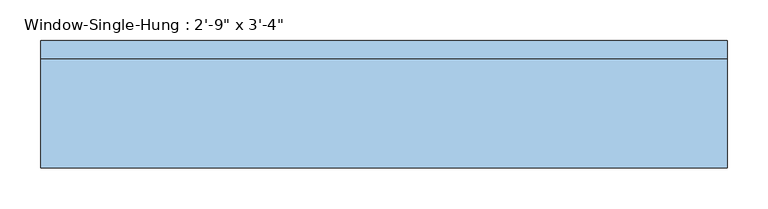
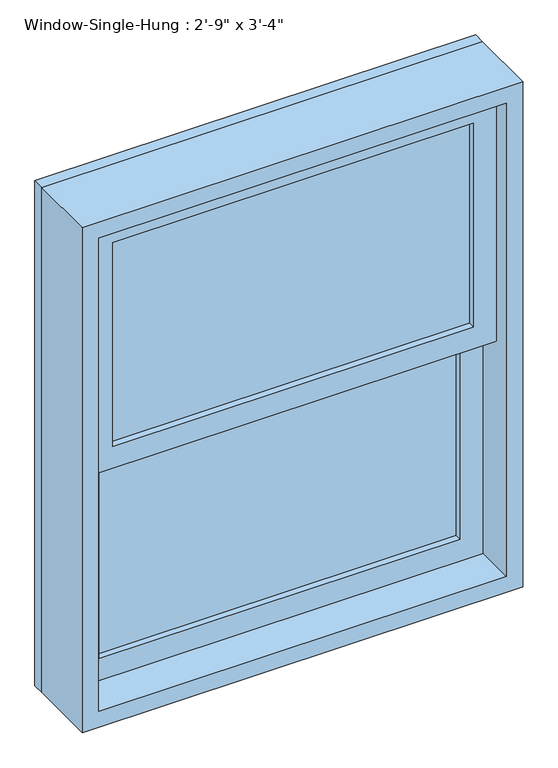
"""IFC4 building model written with IfcOpenShell, lengths in millimetres: window geometry."""

import ifcopenshell
import ifcopenshell.guid

model = None  # the IFC model being written
_history = None  # IfcOwnerHistory: only IFC2X3 demands one
_inside = {}  # id of a spatial element -> (the spatial element, [elements in it])
_under = {}  # id of a project, library or spatial element -> (it, [spatial elements below it])
_declared = {}  # id of a project -> (the project, [libraries it declares])
_typed = {}  # id of a type object -> (the type object, [elements of that type])
_made_of = {}  # id of a material, layer set ... -> (it, [elements and type objects made of it])


def new_model(schema):
    """Start an empty IFC model of exactly this schema.

    Asked for "IFC4X3", IfcOpenShell would pick the latest addendum, in which some entities
    have other attributes; the version numbers below select the first issue.
    IFC2X3 requires an IfcOwnerHistory on every rooted entity: one is made here for all.
    """
    global model, _history
    if schema == "IFC4X3":
        model = ifcopenshell.file(schema_version=(4, 3, 0, 0))
    else:
        model = ifcopenshell.file(schema=schema)
    _inside.clear()
    _under.clear()
    _declared.clear()
    _typed.clear()
    _made_of.clear()
    _history = None
    if model.schema == "IFC2X3":
        org = make("IfcOrganization", Name="unknown")
        user = make(
            "IfcPersonAndOrganization",
            ThePerson=make("IfcPerson", FamilyName="unknown"),
            TheOrganization=org,
        )
        app = make(
            "IfcApplication",
            ApplicationDeveloper=org,
            Version="unknown",
            ApplicationFullName="unknown",
            ApplicationIdentifier="unknown",
        )
        _history = make(
            "IfcOwnerHistory",
            OwningUser=user,
            OwningApplication=app,
            ChangeAction="ADDED",
            CreationDate=0,
        )
    return model


def make(cls, **values):
    """One entity of the class cls with the attributes given. An attribute that is None is left unset."""
    return model.create_entity(
        cls, **{name: value for name, value in values.items() if value is not None}
    )


def rooted(cls, **values):
    """An entity with a GlobalId (a new one), such as an element, a storey or a relation."""
    return make(cls, GlobalId=ifcopenshell.guid.new(), OwnerHistory=_history, **values)


def si_unit(unit_type, name, prefix=None):
    """IfcSIUnit, for example si_unit("LENGTHUNIT", "METRE", prefix="MILLI")."""
    return make("IfcSIUnit", UnitType=unit_type, Prefix=prefix, Name=name)


def assignment(units):
    """IfcUnitAssignment: the units of a project."""
    return None if units is None else make("IfcUnitAssignment", Units=units)


def point(xyz):
    """IfcCartesianPoint."""
    return None if xyz is None else make("IfcCartesianPoint", Coordinates=xyz)


def direction(xyz):
    """IfcDirection."""
    return None if xyz is None else make("IfcDirection", DirectionRatios=xyz)


def frame(location, z_axis=None, x_axis=None):
    """IfcAxis2Placement3D, a coordinate frame: its origin and axes. An axis left out is left unset."""
    return make(
        "IfcAxis2Placement3D",
        Location=point(location),
        Axis=direction(z_axis),
        RefDirection=direction(x_axis),
    )


def origin():
    """The frame at (0, 0, 0) with its axes left unset."""
    return frame((0.0, 0.0, 0.0))


def place(relative_to, where):
    """IfcLocalPlacement: puts the frame where relative to a parent placement (None: the world)."""
    return make(
        "IfcLocalPlacement", PlacementRelTo=relative_to, RelativePlacement=where
    )


def context(
    kind, dimensions, precision=None, world=None, true_north=None, identifier=None
):
    """IfcGeometricRepresentationContext, for example the 3D "Model" context."""
    return make(
        "IfcGeometricRepresentationContext",
        ContextIdentifier=identifier,
        ContextType=kind,
        CoordinateSpaceDimension=dimensions,
        Precision=precision,
        WorldCoordinateSystem=world,
        TrueNorth=true_north,
    )


def project(units=None, contexts=None):
    """IfcProject with its units and contexts."""
    return rooted(
        "IfcProject",
        Name="project",
        RepresentationContexts=contexts,
        UnitsInContext=assignment(units),
    )


def spatial(cls, under=None, at=None, **own):
    """A site, building, storey or space (cls), placed at a placement, below another one or the project."""
    s = rooted(cls, ObjectPlacement=at, **own)
    if under is not None:
        _under.setdefault(under.id(), (under, []))[1].append(s)
    return s


def polyline(points):
    """IfcPolyline through the points."""
    return make("IfcPolyline", Points=[point(p) for p in points])


def outline(outer, holes=None, kind="AREA"):
    """IfcArbitraryClosedProfileDef: a profile drawn as a closed curve; with holes, ...WithVoids."""
    if holes is None:
        return make("IfcArbitraryClosedProfileDef", ProfileType=kind, OuterCurve=outer)
    return make(
        "IfcArbitraryProfileDefWithVoids",
        ProfileType=kind,
        OuterCurve=outer,
        InnerCurves=holes,
    )


def extrude(swept, where, along, depth):
    """IfcExtrudedAreaSolid: the profile swept, set in the frame where, extruded along a direction by depth."""
    return make(
        "IfcExtrudedAreaSolid",
        SweptArea=swept,
        Position=where,
        ExtrudedDirection=direction(along),
        Depth=depth,
    )


def shape(context_of_items, identifier, shape_type, items):
    """IfcShapeRepresentation: the items that make up one representation, for example the "Body"."""
    return make(
        "IfcShapeRepresentation",
        ContextOfItems=context_of_items,
        RepresentationIdentifier=identifier,
        RepresentationType=shape_type,
        Items=items,
    )


def source(mapping_origin, context_of_items, identifier, shape_type, items):
    """IfcRepresentationMap: a shape defined once, which mapped items show again and again."""
    return make(
        "IfcRepresentationMap",
        MappingOrigin=mapping_origin,
        MappedRepresentation=shape(context_of_items, identifier, shape_type, items),
    )


def transform(
    local_origin,
    x_axis=None,
    y_axis=None,
    z_axis=None,
    scale=None,
    scale2=None,
    scale3=None,
    uniform=True,
):
    """IfcCartesianTransformationOperator3D, or its non-uniform kind. x_axis, y_axis, z_axis: its Axis1, 2, 3."""
    if uniform:
        return make(
            "IfcCartesianTransformationOperator3D",
            Axis1=direction(x_axis),
            Axis2=direction(y_axis),
            LocalOrigin=point(local_origin),
            Scale=scale,
            Axis3=direction(z_axis),
        )
    return make(
        "IfcCartesianTransformationOperator3DnonUniform",
        Axis1=direction(x_axis),
        Axis2=direction(y_axis),
        LocalOrigin=point(local_origin),
        Scale=scale,
        Axis3=direction(z_axis),
        Scale2=scale2,
        Scale3=scale3,
    )


def mapped(mapping_source, mapping_target):
    """IfcMappedItem: shows the shape of a source again, moved by a transform."""
    return make(
        "IfcMappedItem", MappingSource=mapping_source, MappingTarget=mapping_target
    )


def made_of(thing, what):
    """Note that an element or type object is made of a material, layer set ...; save() writes the relation."""
    if what is not None:
        _made_of.setdefault(what.id(), (what, []))[1].append(thing)
    return thing


def element(
    cls,
    number,
    at=None,
    inside=None,
    cuts=None,
    type_object=None,
    material=None,
    context=None,
    identifier="Body",
    shape_type=None,
    held_by="IfcProductDefinitionShape",
    body=None,
    shapes=None,
    **own,
):
    """One element of the class cls, such as IfcWall. Its Tag is "e" and its number.

    at: its placement. inside: the storey or other place that contains it. cuts: it is an
    opening in that element (IfcRelVoidsElement). A single representation is given by context,
    identifier, shape_type and body (its items); several are given by shapes. held_by: the class
    of the entity that holds the representations. save() writes the other relations.
    """
    e = rooted(cls, Tag="e%d" % number, ObjectPlacement=at, **own)
    if body is not None:
        shapes = [shape(context, identifier, shape_type, body)]
    if shapes is not None:
        e.Representation = make(held_by, Representations=shapes)
    if inside is not None:
        _inside.setdefault(inside.id(), (inside, []))[1].append(e)
    if cuts is not None:
        rooted(
            "IfcRelVoidsElement", RelatingBuildingElement=cuts, RelatedOpeningElement=e
        )
    if type_object is not None:
        _typed.setdefault(type_object.id(), (type_object, []))[1].append(e)
    return made_of(e, material)


def aggregate(whole, parts):
    """IfcRelAggregates: a whole, such as a stair, and the parts it consists of."""
    return rooted("IfcRelAggregates", RelatingObject=whole, RelatedObjects=parts)


def save(model, path):
    """Write the relations noted so far, then the file.

    IfcRelAggregates (storeys below a building ...), IfcRelContainedInSpatialStructure (elements
    in a storey), IfcRelDefinesByType, IfcRelAssociatesMaterial and IfcRelDeclares: one each for
    every whole, place, type object, material and project.
    """
    for whole, parts in _under.values():
        aggregate(whole, parts)
    for where, things in _inside.values():
        rooted(
            "IfcRelContainedInSpatialStructure",
            RelatedElements=things,
            RelatingStructure=where,
        )
    for kind, things in _typed.values():
        rooted("IfcRelDefinesByType", RelatedObjects=things, RelatingType=kind)
    for what, things in _made_of.values():
        rooted("IfcRelAssociatesMaterial", RelatedObjects=things, RelatingMaterial=what)
    for by, libraries in _declared.values():
        rooted("IfcRelDeclares", RelatingContext=by, RelatedDefinitions=libraries)
    model.write(path)


def window_d23c6517(model_context):
    return source(origin(), model_context, "Body", "SweptSolid", [
        extrude(outline(polyline([(342.9, 1.5875), (-342.9, 1.5875), (-342.9, 7.9375), (342.9, 7.9375), (342.9, 1.5875)])), frame((0.0, 0.0, 990.6), z_axis=(0.0, 0.0, 1.0), x_axis=(1.0, 0.0, 0.0)), (0.0, 0.0, 1.0), 409.575),
        extrude(outline(polyline([(-342.9, 14.2875), (-342.9, 20.6375), (342.9, 20.6375), (342.9, 14.2875), (-342.9, 14.2875)])), frame((0.0, 0.0, 990.6), z_axis=(0.0, 0.0, 1.0), x_axis=(1.0, 0.0, 0.0)), (0.0, 0.0, 1.0), 409.575),
        extrude(outline(polyline([(342.9, -42.8625), (-342.9, -42.8625), (-342.9, -36.5125), (342.9, -36.5125), (342.9, -42.8625)])), frame((0.0, 0.0, 1444.625), z_axis=(0.0, 0.0, 1.0), x_axis=(1.0, 0.0, 0.0)), (0.0, 0.0, 1.0), 409.575),
        extrude(outline(polyline([(-342.9, -30.1625), (-342.9, -23.8125), (342.9, -23.8125), (342.9, -30.1625), (-342.9, -30.1625)])), frame((0.0, 0.0, 1444.625), z_axis=(0.0, 0.0, 1.0), x_axis=(1.0, 0.0, 0.0)), (0.0, 0.0, 1.0), 409.575),
        extrude(outline(polyline([(1444.625, 387.35), (1444.625, -387.35), (946.15, -387.35), (946.15, 387.35), (1444.625, 387.35)]), holes=[polyline([(1400.175, -342.9), (1400.175, 342.9), (990.6, 342.9), (990.6, -342.9), (1400.175, -342.9)])]), frame((0.0, -11.1125, 0.0), z_axis=(0.0, 1.0, 0.0), x_axis=(0.0, 0.0, 1.0)), (0.0, 0.0, 1.0), 44.45),
        extrude(outline(polyline([(1898.65, 387.35), (1898.65, -387.35), (1400.175, -387.35), (1400.175, 387.35), (1898.65, 387.35)]), holes=[polyline([(1854.2, -342.9), (1854.2, 342.9), (1444.625, 342.9), (1444.625, -342.9), (1854.2, -342.9)])]), frame((0.0, -55.5625, 0.0), z_axis=(0.0, 1.0, 0.0), x_axis=(0.0, 0.0, 1.0)), (0.0, 0.0, 1.0), 44.45),
        extrude(outline(polyline([(1930.4, 419.1), (1930.4, -419.1), (914.4, -419.1), (914.4, 419.1), (1930.4, 419.1)]), holes=[polyline([(1898.65, -387.35), (1898.65, 387.35), (946.15, 387.35), (946.15, -387.35), (1898.65, -387.35)])]), frame((0.0, -87.3125, 0.0), z_axis=(0.0, 1.0, 0.0), x_axis=(0.0, 0.0, 1.0)), (0.0, 0.0, 1.0), 133.35),
        extrude(outline(polyline([(1930.4, 419.1), (1930.4, -419.1), (914.4, -419.1), (914.4, 419.1), (1930.4, 419.1)]), holes=[polyline([(1911.35, 400.05), (933.45, 400.05), (933.45, -400.05), (1911.35, -400.05), (1911.35, 400.05)])]), frame((0.0, 46.0375, 0.0), z_axis=(0.0, 1.0, 0.0), x_axis=(0.0, 0.0, 1.0)), (0.0, 0.0, 1.0), 22.225),
    ])


if __name__ == "__main__":
    model = new_model("IFC4")
    model_context = context("Model", 3, world=origin())
    ifc_project = project(units=[si_unit("LENGTHUNIT", "METRE", prefix="MILLI")], contexts=[model_context])
    site = spatial("IfcSite", under=ifc_project)
    building = spatial("IfcBuilding", under=site)
    placement = place(None, origin())
    window_shape = window_d23c6517(model_context)
    element("IfcWindow", 1, ObjectType="Window-Single-Hung : 2'-9\" x 3'-4\"", at=placement, inside=building, context=model_context, shape_type="MappedRepresentation", body=[
        mapped(window_shape, transform((0.0, 0.0, 0.0), x_axis=(1.0, 0.0, 0.0), y_axis=(0.0, 1.0, 0.0), z_axis=(0.0, 0.0, 1.0))),
    ])
    save(model, "model.ifc")

# Revit data of these elements
# Type "Window-Single-Hung : 2'-9\" x 3'-4\""
#   Type Mark = "22"
#   Fire Rating = "0.5h"
#   Construction Type Id = "DG-DR"
#   Assembly Code = "B2020100"
#   Analytic Construction = "Double glazing - domestic"
#   Wall Thickness [instance default] = 0' - 6"
#   Window Inset [instance default] = 0' - 0"
#   Visual Light Transmittance = 0.81
#   Thermal Resistance (R) = 0.319569 (m²·K)/W
#   Solar Heat Gain Coefficient = 0.76
#   Muntin Width = 2' - 3"
#   Muntin Height = 1' - 4 1/8"
#   Interior Wall Closure [instance default] = 0' - 1 1/2"
#   Rough Width = 2' - 9 1/2"
#   Rough Height = 3' - 4 1/2"
#   Frame Extension [instance default] = 0' - 1 1/4"
#   Exterior Wall Closure [instance default] = 0' - 0 1/2"
#   Extension Jamb [instance default] = 0' - 1 1/2"
#   Heat Transfer Coefficient (U) = 3.12929 W/(m²·K)
#   Height = 3' - 4"
#   Width = 2' - 9"
#   Top Muntin Visibility = yes
#   Indicator Visibility [instance default] = yes
#   Extension Jamb Visibility [instance default] = yes
#   Interior Trim Visibility [instance default] = yes
#   Exterior Trim Visibility [instance default] = yes
#   Bottom Muntin Visibility = yes
#   Muntin Pattern = Muntin Pattern_2x2 : Muntin Pattern_2x2
#   Interior Trim Material = Wood - Stained
#   Interior Trim = Trim-Window-Interior-Flat : Picture Frame
#   Exterior Trim Material = Clad - White
#   Exterior Trim = Trim-Window-Exterior-Flat : with Sill
#   Glass Panel Material = Glass
#   Exterior Frame Material = Clad - White
#   Interior Frame Material = Wood - Stained
#   Wall Closure = (empty or 0)
# Element 1 (IfcWindow, "Window-Single-Hung : 2'-9\" x 3'-4\"")
#   Wall Thickness = 0' - 5 3/8"
#   Extension Jamb = 0' - 0 7/8"
#   Materials on its faces: "Wood - Stained", "Glass", "Clad - White"
# Materials
#   "Wood - Stained": class "Wood", colour RGB 224 178 126, transparency 0, Cost = 0
#   "Clad - White": class "Wood", colour RGB 242 242 238, transparency 0, Cost = 0
#   "Glass": class "Glass", colour RGB 0 128 192, transparency 0.75, Description = "Soda Lime Glass", Cost = 0
